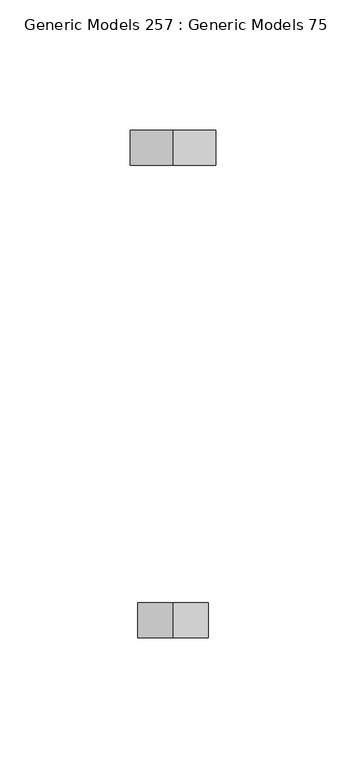
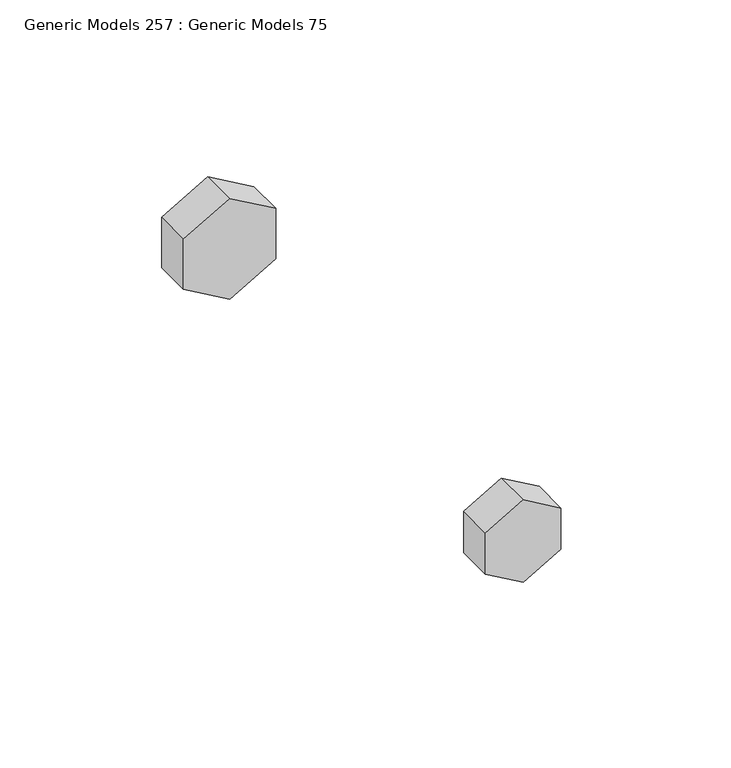
"""IFC4 building model written with IfcOpenShell, lengths in millimetres: proxy geometry, Generic Models 257 : Generic Models 75."""

from ifc_helpers import new_model, si_unit, frame, origin, place, context, project, spatial, polyline, outline, extrude, source, transform, mapped, element, save


def generic_models_257_generic_models_75_470e363e(model_context):
    return source(origin(), model_context, "Body", "SweptSolid", [
        extrude(outline(polyline([(266525.375, 32004.6193618), (266544.425, 32004.6193618), (266553.95, 31988.1215778), (266544.425, 31971.6237939), (266525.375, 31971.6237939), (266515.85, 31988.1215778), (266525.375, 32004.6193618)])), frame((0.0, 36491.5582942, 0.0), z_axis=(0.0, 1.0, 0.0), x_axis=(0.0, 0.0, 1.0)), (0.0, 0.0, 1.0), 13.49375),
        extrude(outline(polyline([(266542.5078422, 31974.6312024), (266526.9304985, 31974.6312024), (266519.1418266, 31988.1215778), (266526.9304985, 32001.6119532), (266542.5078422, 32001.6119532), (266550.2965141, 31988.1215778), (266542.5078422, 31974.6312024)])), frame((0.0, 36309.7895442, 0.0), z_axis=(0.0, 1.0, 0.0), x_axis=(0.0, 0.0, 1.0)), (0.0, 0.0, 1.0), 13.49375),
    ])


if __name__ == "__main__":
    model = new_model("IFC4")
    model_context = context("Model", 3, world=origin())
    ifc_project = project(units=[si_unit("LENGTHUNIT", "METRE", prefix="MILLI")], contexts=[model_context])
    site = spatial("IfcSite", under=ifc_project)
    building = spatial("IfcBuilding", under=site)
    placement = place(None, origin())
    generic_models_257_generic_models_75_shape = generic_models_257_generic_models_75_470e363e(model_context)
    element("IfcBuildingElementProxy", 1, Name="Generic Models 257 : Generic Models 75", ObjectType="Generic Models 257 : Generic Models 75", at=placement, inside=building, context=model_context, shape_type="MappedRepresentation", body=[
        mapped(generic_models_257_generic_models_75_shape, transform((0.0, 0.0, 0.0), x_axis=(1.0, 0.0, 0.0), y_axis=(0.0, 1.0, 0.0), z_axis=(0.0, 0.0, 1.0))),
    ])
    save(model, "model.ifc")

# Revit data of these elements
# Element 1 (IfcBuildingElementProxy, "Generic Models 257 : Generic Models 75")
#   Materials on its faces: "5/8\" GALV. THRU BOLTS"
# Materials
#   "5/8\" GALV. THRU BOLTS": class "Generic", colour RGB 255 0 255, transparency 0, Cost = 0
